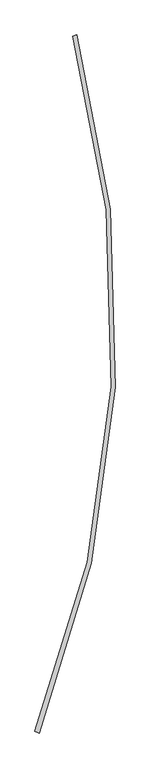
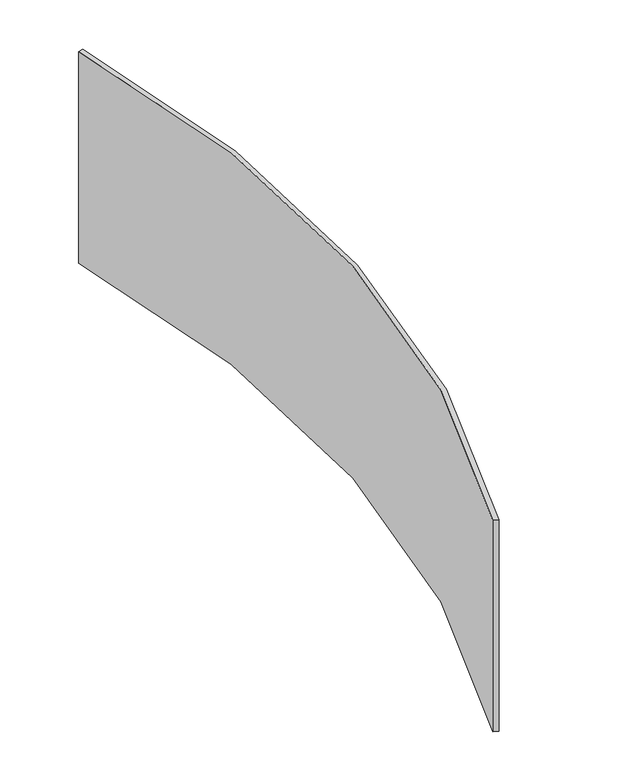
"""IFC4 building model written with IfcOpenShell, lengths in millimetres: railing geometry, Barandillas 1 : Barandillas 1."""

from ifc_helpers import new_model, si_unit, point, frame, frame_2d, origin, place, context, project, spatial, polyline, circle_curve, trimmed, segment, composite_curve, outline, extrude, source, transform, mapped, element, save


def railing_a4b388ec(model_context):
    return source(origin(), model_context, "Body", "SweptSolid", [
        extrude(outline(composite_curve([segment(polyline([(-219.9286151, 3647.9966808), (-202.089662, 3652.9847374)]), True, "CONTINUOUS"), segment(trimmed(circle_curve(frame_2d((-4777.5732657, 2383.9428343)), 4748.2120383), [point((-202.089662, 3652.9847374))], [point((-364.4540748, 631.8308041))], False, "CARTESIAN"), True, "CONTINUOUS"), segment(polyline([(-364.4540748, 631.8308041), (-383.0202456, 639.2670194)]), True, "CONTINUOUS"), segment(trimmed(circle_curve(frame_2d((-4739.6561895, 2384.2085657)), 4693.0904261), [point((-383.0202456, 639.2670194))], [point((-219.9286151, 3647.9966808))], True, "CARTESIAN"), True, "CONTINUOUS")], self_intersect=False)), frame((0.0, 0.0, 6100.0), z_axis=(0.0, 0.0, 1.0), x_axis=(1.0, 0.0, 0.0)), (0.0, 0.0, 1.0), 850.0),
    ])


if __name__ == "__main__":
    model = new_model("IFC4")
    model_context = context("Model", 3, world=origin())
    ifc_project = project(units=[si_unit("LENGTHUNIT", "METRE", prefix="MILLI")], contexts=[model_context])
    site = spatial("IfcSite", under=ifc_project)
    building = spatial("IfcBuilding", under=site)
    placement = place(None, origin())
    railing_shape = railing_a4b388ec(model_context)
    element("IfcRailing", 1, ObjectType="Barandillas 1 : Barandillas 1", at=placement, inside=building, context=model_context, shape_type="MappedRepresentation", body=[
        mapped(railing_shape, transform((0.0, 0.0, 0.0), x_axis=(1.0, 0.0, 0.0), y_axis=(0.0, 1.0, 0.0), z_axis=(0.0, 0.0, 1.0))),
    ])
    save(model, "model.ifc")

# Revit data of these elements
# Element 1 (IfcRailing, "Barandillas 1 : Barandillas 1")
#   Materials on its faces: "VIDRIO"
# Materials
#   "VIDRIO": class "Genérico", colour RGB 120 120 120, transparency 0, Cost = 0
